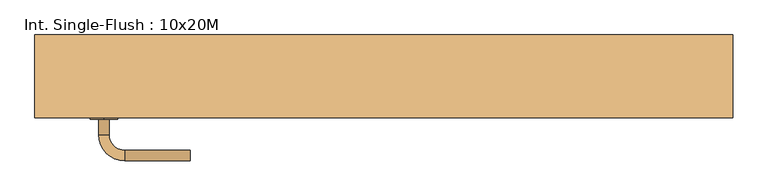
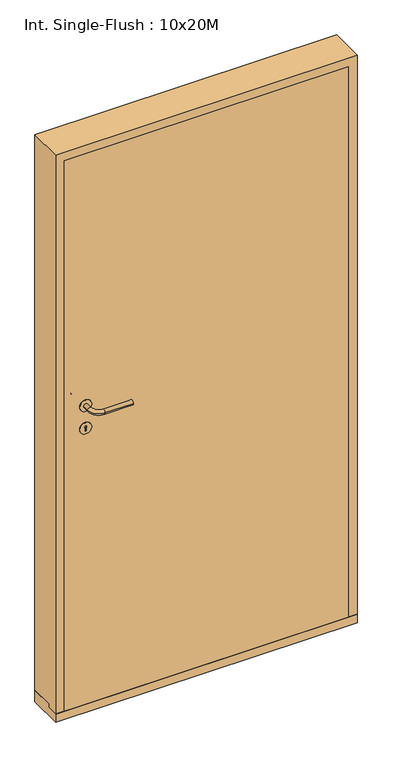
"""IFC4 building model written with IfcOpenShell, lengths in millimetres: door geometry, Int. Single-Flush : 10x20M."""

import ifcopenshell
import ifcopenshell.guid

model = None  # the IFC model being written
_history = None  # IfcOwnerHistory: only IFC2X3 demands one
_inside = {}  # id of a spatial element -> (the spatial element, [elements in it])
_under = {}  # id of a project, library or spatial element -> (it, [spatial elements below it])
_declared = {}  # id of a project -> (the project, [libraries it declares])
_typed = {}  # id of a type object -> (the type object, [elements of that type])
_made_of = {}  # id of a material, layer set ... -> (it, [elements and type objects made of it])


def new_model(schema):
    """Start an empty IFC model of exactly this schema.

    Asked for "IFC4X3", IfcOpenShell would pick the latest addendum, in which some entities
    have other attributes; the version numbers below select the first issue.
    IFC2X3 requires an IfcOwnerHistory on every rooted entity: one is made here for all.
    """
    global model, _history
    if schema == "IFC4X3":
        model = ifcopenshell.file(schema_version=(4, 3, 0, 0))
    else:
        model = ifcopenshell.file(schema=schema)
    _inside.clear()
    _under.clear()
    _declared.clear()
    _typed.clear()
    _made_of.clear()
    _history = None
    if model.schema == "IFC2X3":
        org = make("IfcOrganization", Name="unknown")
        user = make(
            "IfcPersonAndOrganization",
            ThePerson=make("IfcPerson", FamilyName="unknown"),
            TheOrganization=org,
        )
        app = make(
            "IfcApplication",
            ApplicationDeveloper=org,
            Version="unknown",
            ApplicationFullName="unknown",
            ApplicationIdentifier="unknown",
        )
        _history = make(
            "IfcOwnerHistory",
            OwningUser=user,
            OwningApplication=app,
            ChangeAction="ADDED",
            CreationDate=0,
        )
    return model


def make(cls, **values):
    """One entity of the class cls with the attributes given. An attribute that is None is left unset."""
    return model.create_entity(
        cls, **{name: value for name, value in values.items() if value is not None}
    )


def rooted(cls, **values):
    """An entity with a GlobalId (a new one), such as an element, a storey or a relation."""
    return make(cls, GlobalId=ifcopenshell.guid.new(), OwnerHistory=_history, **values)


def si_unit(unit_type, name, prefix=None):
    """IfcSIUnit, for example si_unit("LENGTHUNIT", "METRE", prefix="MILLI")."""
    return make("IfcSIUnit", UnitType=unit_type, Prefix=prefix, Name=name)


def assignment(units):
    """IfcUnitAssignment: the units of a project."""
    return None if units is None else make("IfcUnitAssignment", Units=units)


def point(xyz):
    """IfcCartesianPoint."""
    return None if xyz is None else make("IfcCartesianPoint", Coordinates=xyz)


def direction(xyz):
    """IfcDirection."""
    return None if xyz is None else make("IfcDirection", DirectionRatios=xyz)


def frame(location, z_axis=None, x_axis=None):
    """IfcAxis2Placement3D, a coordinate frame: its origin and axes. An axis left out is left unset."""
    return make(
        "IfcAxis2Placement3D",
        Location=point(location),
        Axis=direction(z_axis),
        RefDirection=direction(x_axis),
    )


def frame_2d(location, x_axis=None):
    """IfcAxis2Placement2D, a coordinate frame in the plane: its origin and x axis."""
    return make(
        "IfcAxis2Placement2D", Location=point(location), RefDirection=direction(x_axis)
    )


def origin():
    """The frame at (0, 0, 0) with its axes left unset."""
    return frame((0.0, 0.0, 0.0))


def place(relative_to, where):
    """IfcLocalPlacement: puts the frame where relative to a parent placement (None: the world)."""
    return make(
        "IfcLocalPlacement", PlacementRelTo=relative_to, RelativePlacement=where
    )


def context(
    kind, dimensions, precision=None, world=None, true_north=None, identifier=None
):
    """IfcGeometricRepresentationContext, for example the 3D "Model" context."""
    return make(
        "IfcGeometricRepresentationContext",
        ContextIdentifier=identifier,
        ContextType=kind,
        CoordinateSpaceDimension=dimensions,
        Precision=precision,
        WorldCoordinateSystem=world,
        TrueNorth=true_north,
    )


def project(units=None, contexts=None):
    """IfcProject with its units and contexts."""
    return rooted(
        "IfcProject",
        Name="project",
        RepresentationContexts=contexts,
        UnitsInContext=assignment(units),
    )


def spatial(cls, under=None, at=None, **own):
    """A site, building, storey or space (cls), placed at a placement, below another one or the project."""
    s = rooted(cls, ObjectPlacement=at, **own)
    if under is not None:
        _under.setdefault(under.id(), (under, []))[1].append(s)
    return s


def polyline(points):
    """IfcPolyline through the points."""
    return make("IfcPolyline", Points=[point(p) for p in points])


def circle_curve(where, radius):
    """IfcCircle in the frame where."""
    return make("IfcCircle", Position=where, Radius=radius)


def ellipse_curve(where, semi_axis1, semi_axis2):
    """IfcEllipse in the frame where."""
    return make(
        "IfcEllipse", Position=where, SemiAxis1=semi_axis1, SemiAxis2=semi_axis2
    )


def trimmed(basis, trim1, trim2, sense, master):
    """IfcTrimmedCurve: the piece of a basis curve between two trims."""
    return make(
        "IfcTrimmedCurve",
        BasisCurve=basis,
        Trim1=trim1,
        Trim2=trim2,
        SenseAgreement=sense,
        MasterRepresentation=master,
    )


def segment(curve, same_sense, transition):
    """IfcCompositeCurveSegment."""
    return make(
        "IfcCompositeCurveSegment",
        Transition=transition,
        SameSense=same_sense,
        ParentCurve=curve,
    )


def composite_curve(segments, self_intersect=None):
    """IfcCompositeCurve: segments joined end to end."""
    return make("IfcCompositeCurve", Segments=segments, SelfIntersect=self_intersect)


def outline(outer, holes=None, kind="AREA"):
    """IfcArbitraryClosedProfileDef: a profile drawn as a closed curve; with holes, ...WithVoids."""
    if holes is None:
        return make("IfcArbitraryClosedProfileDef", ProfileType=kind, OuterCurve=outer)
    return make(
        "IfcArbitraryProfileDefWithVoids",
        ProfileType=kind,
        OuterCurve=outer,
        InnerCurves=holes,
    )


def extrude(swept, where, along, depth):
    """IfcExtrudedAreaSolid: the profile swept, set in the frame where, extruded along a direction by depth."""
    return make(
        "IfcExtrudedAreaSolid",
        SweptArea=swept,
        Position=where,
        ExtrudedDirection=direction(along),
        Depth=depth,
    )


def faces_of(points, faces, orient=None, outer=None):
    """IfcFace entities. A face is a list of loops; a loop is a list of indices into points, from 0.

    orient and outer hold one flag for each loop. By default every Orientation is true, the
    first loop of a face is its IfcFaceOuterBound and the others are IfcFaceBound.
    """
    made = []
    for i, loops in enumerate(faces):
        bounds = []
        for j, loop in enumerate(loops):
            is_outer = j == 0 if outer is None else outer[i][j]
            bounds.append(
                make(
                    "IfcFaceOuterBound" if is_outer else "IfcFaceBound",
                    Bound=make("IfcPolyLoop", Polygon=[points[k] for k in loop]),
                    Orientation=True if orient is None else orient[i][j],
                )
            )
        made.append(make("IfcFace", Bounds=bounds))
    return made


def faceted_brep(points, faces, orient=None, outer=None, voids=None):
    """IfcFacetedBrep: a solid bounded by flat faces; with voids (closed shells), ...WithVoids."""
    shared = [point(p) for p in points]
    hull = make("IfcClosedShell", CfsFaces=faces_of(shared, faces, orient, outer))
    if voids is None:
        return make("IfcFacetedBrep", Outer=hull)
    return make(
        "IfcFacetedBrepWithVoids",
        Outer=hull,
        Voids=[
            make(cls, CfsFaces=faces_of(shared, fs, o, b)) for cls, fs, o, b in voids
        ],
    )


def shape(context_of_items, identifier, shape_type, items):
    """IfcShapeRepresentation: the items that make up one representation, for example the "Body"."""
    return make(
        "IfcShapeRepresentation",
        ContextOfItems=context_of_items,
        RepresentationIdentifier=identifier,
        RepresentationType=shape_type,
        Items=items,
    )


def source(mapping_origin, context_of_items, identifier, shape_type, items):
    """IfcRepresentationMap: a shape defined once, which mapped items show again and again."""
    return make(
        "IfcRepresentationMap",
        MappingOrigin=mapping_origin,
        MappedRepresentation=shape(context_of_items, identifier, shape_type, items),
    )


def transform(
    local_origin,
    x_axis=None,
    y_axis=None,
    z_axis=None,
    scale=None,
    scale2=None,
    scale3=None,
    uniform=True,
):
    """IfcCartesianTransformationOperator3D, or its non-uniform kind. x_axis, y_axis, z_axis: its Axis1, 2, 3."""
    if uniform:
        return make(
            "IfcCartesianTransformationOperator3D",
            Axis1=direction(x_axis),
            Axis2=direction(y_axis),
            LocalOrigin=point(local_origin),
            Scale=scale,
            Axis3=direction(z_axis),
        )
    return make(
        "IfcCartesianTransformationOperator3DnonUniform",
        Axis1=direction(x_axis),
        Axis2=direction(y_axis),
        LocalOrigin=point(local_origin),
        Scale=scale,
        Axis3=direction(z_axis),
        Scale2=scale2,
        Scale3=scale3,
    )


def mapped(mapping_source, mapping_target):
    """IfcMappedItem: shows the shape of a source again, moved by a transform."""
    return make(
        "IfcMappedItem", MappingSource=mapping_source, MappingTarget=mapping_target
    )


def made_of(thing, what):
    """Note that an element or type object is made of a material, layer set ...; save() writes the relation."""
    if what is not None:
        _made_of.setdefault(what.id(), (what, []))[1].append(thing)
    return thing


def element(
    cls,
    number,
    at=None,
    inside=None,
    cuts=None,
    type_object=None,
    material=None,
    context=None,
    identifier="Body",
    shape_type=None,
    held_by="IfcProductDefinitionShape",
    body=None,
    shapes=None,
    **own,
):
    """One element of the class cls, such as IfcWall. Its Tag is "e" and its number.

    at: its placement. inside: the storey or other place that contains it. cuts: it is an
    opening in that element (IfcRelVoidsElement). A single representation is given by context,
    identifier, shape_type and body (its items); several are given by shapes. held_by: the class
    of the entity that holds the representations. save() writes the other relations.
    """
    e = rooted(cls, Tag="e%d" % number, ObjectPlacement=at, **own)
    if body is not None:
        shapes = [shape(context, identifier, shape_type, body)]
    if shapes is not None:
        e.Representation = make(held_by, Representations=shapes)
    if inside is not None:
        _inside.setdefault(inside.id(), (inside, []))[1].append(e)
    if cuts is not None:
        rooted(
            "IfcRelVoidsElement", RelatingBuildingElement=cuts, RelatedOpeningElement=e
        )
    if type_object is not None:
        _typed.setdefault(type_object.id(), (type_object, []))[1].append(e)
    return made_of(e, material)


def aggregate(whole, parts):
    """IfcRelAggregates: a whole, such as a stair, and the parts it consists of."""
    return rooted("IfcRelAggregates", RelatingObject=whole, RelatedObjects=parts)


def save(model, path):
    """Write the relations noted so far, then the file.

    IfcRelAggregates (storeys below a building ...), IfcRelContainedInSpatialStructure (elements
    in a storey), IfcRelDefinesByType, IfcRelAssociatesMaterial and IfcRelDeclares: one each for
    every whole, place, type object, material and project.
    """
    for whole, parts in _under.values():
        aggregate(whole, parts)
    for where, things in _inside.values():
        rooted(
            "IfcRelContainedInSpatialStructure",
            RelatedElements=things,
            RelatingStructure=where,
        )
    for kind, things in _typed.values():
        rooted("IfcRelDefinesByType", RelatedObjects=things, RelatingType=kind)
    for what, things in _made_of.values():
        rooted("IfcRelAssociatesMaterial", RelatedObjects=things, RelatingMaterial=what)
    for by, libraries in _declared.values():
        rooted("IfcRelDeclares", RelatingContext=by, RelatedDefinitions=libraries)
    model.write(path)


def plane_surface(at):
    """IfcPlane: the flat surface through the origin of the frame at, square to its z axis."""
    return make("IfcPlane", Position=at)


def cylinder_surface(at, radius):
    """IfcCylindricalSurface: all points at the distance radius from the z axis of the frame at."""
    return make("IfcCylindricalSurface", Position=at, Radius=radius)


def revolved_surface(curve, axis_point, axis_direction):
    """IfcSurfaceOfRevolution: the curve turned about the line through axis_point along axis_direction."""
    return make(
        "IfcSurfaceOfRevolution",
        SweptCurve=make("IfcArbitraryOpenProfileDef", ProfileType="CURVE", Curve=curve),
        AxisPosition=make("IfcAxis1Placement", Location=point(axis_point), Axis=direction(axis_direction)),
    )


def advanced_brep(points, edges, surfaces, faces):
    """IfcAdvancedBrep: a solid bounded by faces that lie on surfaces and meet in shared edges.

    An edge is (start, end): straight between two places in points (the first is 0);
    or (start, end, curve); or (start, end, curve, False) where it runs against its curve.
    A face is (place in surfaces, loops), or (place, loops, False) where it looks against
    its surface's normal. A loop lists edges by number (the first is 1), with a minus sign
    where the edge is run from its end to its start. The first loop is the outer one.
    """
    corners = [point(p) for p in points]
    vertices = [make("IfcVertexPoint", VertexGeometry=c) for c in corners]
    made = []
    for start, end, *more in edges:
        made.append(
            make(
                "IfcEdgeCurve",
                EdgeStart=vertices[start],
                EdgeEnd=vertices[end],
                EdgeGeometry=more[0] if more else make("IfcPolyline", Points=[corners[start], corners[end]]),
                SameSense=more[1] if len(more) > 1 else True,
            )
        )
    hull = []
    for where, loops, *sense in faces:
        bounds = []
        for j, loop in enumerate(loops):
            ring = [make("IfcOrientedEdge", EdgeElement=made[abs(k) - 1], Orientation=k > 0) for k in loop]
            bounds.append(
                make(
                    "IfcFaceOuterBound" if j == 0 else "IfcFaceBound",
                    Bound=make("IfcEdgeLoop", EdgeList=ring),
                    Orientation=True,
                )
            )
        hull.append(make("IfcAdvancedFace", Bounds=bounds, FaceSurface=surfaces[where], SameSense=sense[0] if sense else True))
    return make("IfcAdvancedBrep", Outer=make("IfcClosedShell", CfsFaces=hull))


def int_single_flush_10x20m_68751a9d(model_context):
    return source(origin(), model_context, "Body", "SolidModel", [
        extrude(outline(composite_curve([segment(trimmed(circle_curve(frame_2d((1090.0, -406.0)), 20.0), [point((1070.0, -406.0))], [point((1110.0, -406.0))], False, "CARTESIAN"), True, "CONTINUOUS"), segment(trimmed(circle_curve(frame_2d((1090.0, -406.0)), 20.0), [point((1110.0, -406.0))], [point((1070.0, -406.0))], False, "CARTESIAN"), True, "CONTINUOUS")], self_intersect=False)), frame((0.0, -62.0, 0.0), z_axis=(0.0, 1.0, 0.0), x_axis=(0.0, 0.0, 1.0)), (0.0, 0.0, 1.0), 2.0),
        advanced_brep(
        [(-413.5, -62.0, 1090.0), (-398.5, -62.0, 1090.0), (-398.5, -84.5, 1090.0), (-413.5, -84.5, 1090.0), (-376.0, -107.0, 1090.0), (-376.0, -122.0, 1090.0), (-281.0, -107.0, 1090.0), (-281.0, -122.0, 1090.0)],
        [
            (0, 1, circle_curve(frame((-406.0, -62.0, 1090.0), z_axis=(0.0, 1.0, 0.0), x_axis=(1.0, 0.0, 0.0)), 7.5)),
            (1, 0, circle_curve(frame((-406.0, -62.0, 1090.0), z_axis=(0.0, 1.0, 0.0), x_axis=(1.0, 0.0, 0.0)), 7.5)),
            (1, 2),
            (2, 3, circle_curve(frame((-406.0, -84.5, 1090.0), z_axis=(0.0, 1.0, 0.0), x_axis=(1.0, 0.0, 0.0)), 7.5)),
            (3, 0),
            (3, 2, circle_curve(frame((-406.0, -84.5, 1090.0), z_axis=(0.0, 1.0, 0.0), x_axis=(1.0, 0.0, 0.0)), 7.5)),
            (4, 5, circle_curve(frame((-376.0, -114.5, 1090.0), z_axis=(-1.0, 0.0, 0.0), x_axis=(0.0, 1.0, 0.0)), 7.5)),
            (5, 3, circle_curve(frame((-376.0, -84.5, 1090.0), z_axis=(0.0, 0.0, -1.0), x_axis=(-1.0, 0.0, 0.0)), 37.5)),
            (2, 4, circle_curve(frame((-376.0, -84.5, 1090.0), z_axis=(0.0, 0.0, 1.0), x_axis=(-1.0, 0.0, 0.0)), 22.5)),
            (5, 4, circle_curve(frame((-376.0, -114.5, 1090.0), z_axis=(-1.0, 0.0, 0.0), x_axis=(0.0, 1.0, 0.0)), 7.5)),
            (4, 6),
            (6, 7, circle_curve(frame((-281.0, -114.5, 1090.0), z_axis=(-1.0, 0.0, 0.0), x_axis=(0.0, 1.0, 0.0)), 7.5)),
            (7, 5),
            (7, 6, circle_curve(frame((-281.0, -114.5, 1090.0), z_axis=(-1.0, 0.0, 0.0), x_axis=(0.0, 1.0, 0.0)), 7.5)),
        ],
        [
            plane_surface(frame((-406.0, -62.0, 1090.0), z_axis=(0.0, 1.0, 0.0), x_axis=(0.0, 0.0, -1.0))),
            cylinder_surface(frame((-406.0, -62.0, 1090.0), z_axis=(0.0, 1.0, 0.0), x_axis=(1.0, 0.0, 0.0)), 7.5),
            revolved_surface(trimmed(ellipse_curve(frame((-406.0, -84.5, 1090.0), z_axis=(0.0, -1.0, 0.0), x_axis=(1.0, 0.0, 0.0)), 7.5, 7.5), [point((-413.5, -84.5, 1090.0))], [point((-398.5, -84.5, 1090.0))], True, "CARTESIAN"), (-376.0, -84.5, 1090.0), (0.0, 0.0, -1.0)),
            revolved_surface(trimmed(ellipse_curve(frame((-406.0, -84.5, 1090.0), z_axis=(0.0, -1.0, 0.0), x_axis=(1.0, 0.0, 0.0)), 7.5, 7.5), [point((-398.5, -84.5, 1090.0))], [point((-413.5, -84.5, 1090.0))], True, "CARTESIAN"), (-376.0, -84.5, 1090.0), (0.0, 0.0, -1.0)),
            cylinder_surface(frame((-376.0, -114.5, 1090.0), z_axis=(-1.0, 0.0, 0.0), x_axis=(0.0, 1.0, 0.0)), 7.5),
            plane_surface(frame((-281.0, -114.5, 1090.0), z_axis=(1.0, 0.0, 0.0), x_axis=(0.0, 0.0, -1.0))),
        ],
        [
            (0, [[1, 2]]),
            (1, [[3, 4, 5, -2]]),
            (1, [[-5, 6, -3, -1]]),
            (2, [[7, 8, -4, 9]]),
            (3, [[10, -9, -6, -8]]),
            (4, [[11, 12, 13, -7]]),
            (4, [[-13, 14, -11, -10]]),
            (5, [[-12, -14]]),
        ],
    ),
        extrude(outline(composite_curve([segment(trimmed(circle_curve(frame_2d((1010.0, -406.0)), 20.0), [point((990.0, -406.0))], [point((1030.0, -406.0))], False, "CARTESIAN"), True, "CONTINUOUS"), segment(trimmed(circle_curve(frame_2d((1010.0, -406.0)), 20.0), [point((1030.0, -406.0))], [point((990.0, -406.0))], False, "CARTESIAN"), True, "CONTINUOUS")], self_intersect=False), holes=[composite_curve([segment(trimmed(circle_curve(frame_2d((1015.0, -406.0)), 3.0), [point((1012.4019238, -407.5))], [point((1012.4019238, -404.5))], True, "CARTESIAN"), True, "CONTINUOUS"), segment(polyline([(1012.4019238, -404.5), (1000.0, -404.5), (1000.0, -407.5), (1012.4019238, -407.5)]), True, "CONTINUOUS")], self_intersect=False)]), frame((0.0, -62.0, 0.0), z_axis=(0.0, 1.0, 0.0), x_axis=(0.0, 0.0, 1.0)), (0.0, 0.0, 1.0), 2.0),
        extrude(outline(composite_curve([segment(trimmed(circle_curve(frame_2d((1090.0, -406.0)), 20.0), [point((1070.0, -406.0))], [point((1110.0, -406.0))], False, "CARTESIAN"), True, "CONTINUOUS"), segment(trimmed(circle_curve(frame_2d((1090.0, -406.0)), 20.0), [point((1110.0, -406.0))], [point((1070.0, -406.0))], False, "CARTESIAN"), True, "CONTINUOUS")], self_intersect=False)), frame((0.0, -20.0, 0.0), z_axis=(0.0, 1.0, 0.0), x_axis=(0.0, 0.0, 1.0)), (0.0, 0.0, 1.0), 2.0),
        advanced_brep(
        [(-413.5, -18.0, 1090.0), (-398.5, -18.0, 1090.0), (-413.5, 4.5, 1090.0), (-398.5, 4.5, 1090.0), (-376.0, 27.0, 1090.0), (-376.0, 42.0, 1090.0), (-281.0, 42.0, 1090.0), (-281.0, 27.0, 1090.0)],
        [
            (0, 1, circle_curve(frame((-406.0, -18.0, 1090.0), z_axis=(0.0, -1.0, 0.0), x_axis=(1.0, 0.0, 0.0)), 7.5)),
            (1, 0, circle_curve(frame((-406.0, -18.0, 1090.0), z_axis=(0.0, -1.0, 0.0), x_axis=(1.0, 0.0, 0.0)), 7.5)),
            (0, 2),
            (2, 3, circle_curve(frame((-406.0, 4.5, 1090.0), z_axis=(0.0, -1.0, 0.0), x_axis=(1.0, 0.0, 0.0)), 7.5)),
            (3, 1),
            (3, 2, circle_curve(frame((-406.0, 4.5, 1090.0), z_axis=(0.0, -1.0, 0.0), x_axis=(1.0, 0.0, 0.0)), 7.5)),
            (4, 3, circle_curve(frame((-376.0, 4.5, 1090.0), z_axis=(0.0, 0.0, 1.0), x_axis=(-1.0, 0.0, 0.0)), 22.5)),
            (2, 5, circle_curve(frame((-376.0, 4.5, 1090.0), z_axis=(0.0, 0.0, -1.0), x_axis=(-1.0, 0.0, 0.0)), 37.5)),
            (5, 4, circle_curve(frame((-376.0, 34.5, 1090.0), z_axis=(-1.0, 0.0, 0.0), x_axis=(0.0, -1.0, 0.0)), 7.5)),
            (4, 5, circle_curve(frame((-376.0, 34.5, 1090.0), z_axis=(-1.0, 0.0, 0.0), x_axis=(0.0, -1.0, 0.0)), 7.5)),
            (5, 6),
            (6, 7, circle_curve(frame((-281.0, 34.5, 1090.0), z_axis=(-1.0, 0.0, 0.0), x_axis=(0.0, -1.0, 0.0)), 7.5)),
            (7, 4),
            (7, 6, circle_curve(frame((-281.0, 34.5, 1090.0), z_axis=(-1.0, 0.0, 0.0), x_axis=(0.0, -1.0, 0.0)), 7.5)),
        ],
        [
            plane_surface(frame((-406.0, -18.0, 1090.0), z_axis=(0.0, -1.0, 0.0), x_axis=(0.0, 0.0, -1.0))),
            cylinder_surface(frame((-406.0, -18.0, 1090.0), z_axis=(0.0, -1.0, 0.0), x_axis=(1.0, 0.0, 0.0)), 7.5),
            revolved_surface(trimmed(ellipse_curve(frame((-406.0, 4.5, 1090.0), z_axis=(0.0, -1.0, 0.0), x_axis=(1.0, 0.0, 0.0)), 7.5, 7.5), [point((-413.5, 4.5, 1090.0))], [point((-398.5, 4.5, 1090.0))], True, "CARTESIAN"), (-376.0, 4.5, 1090.0), (0.0, 0.0, -1.0)),
            revolved_surface(trimmed(ellipse_curve(frame((-406.0, 4.5, 1090.0), z_axis=(0.0, -1.0, 0.0), x_axis=(1.0, 0.0, 0.0)), 7.5, 7.5), [point((-398.5, 4.5, 1090.0))], [point((-413.5, 4.5, 1090.0))], True, "CARTESIAN"), (-376.0, 4.5, 1090.0), (0.0, 0.0, -1.0)),
            cylinder_surface(frame((-376.0, 34.5, 1090.0), z_axis=(-1.0, 0.0, 0.0), x_axis=(0.0, -1.0, 0.0)), 7.5),
            plane_surface(frame((-281.0, 34.5, 1090.0), z_axis=(1.0, 0.0, 0.0), x_axis=(0.0, 0.0, -1.0))),
        ],
        [
            (0, [[1, 2]]),
            (1, [[-1, 3, 4, 5]]),
            (1, [[-2, -5, 6, -3]]),
            (2, [[7, -4, 8, 9]]),
            (3, [[-8, -6, -7, 10]]),
            (4, [[-9, 11, 12, 13]]),
            (4, [[-10, -13, 14, -11]]),
            (5, [[-14, -12]]),
        ],
    ),
        extrude(outline(composite_curve([segment(trimmed(circle_curve(frame_2d((1010.0, -406.0)), 20.0), [point((990.0, -406.0))], [point((1030.0, -406.0))], False, "CARTESIAN"), True, "CONTINUOUS"), segment(trimmed(circle_curve(frame_2d((1010.0, -406.0)), 20.0), [point((1030.0, -406.0))], [point((990.0, -406.0))], False, "CARTESIAN"), True, "CONTINUOUS")], self_intersect=False), holes=[composite_curve([segment(trimmed(circle_curve(frame_2d((1015.0, -406.0)), 3.0), [point((1012.4019238, -407.5))], [point((1012.4019238, -404.5))], True, "CARTESIAN"), True, "CONTINUOUS"), segment(polyline([(1012.4019238, -404.5), (1000.0, -404.5), (1000.0, -407.5), (1012.4019238, -407.5)]), True, "CONTINUOUS")], self_intersect=False)]), frame((0.0, -20.0, 0.0), z_axis=(0.0, 1.0, 0.0), x_axis=(0.0, 0.0, 1.0)), (0.0, 0.0, 1.0), 2.0),
        extrude(outline(polyline([(476.0, -20.0), (476.0, -60.0), (-476.0, -60.0), (-476.0, -20.0), (476.0, -20.0)])), frame((0.0, 0.0, 30.0), z_axis=(0.0, 0.0, 1.0), x_axis=(1.0, 0.0, 0.0)), (0.0, 0.0, 1.0), 1952.0),
        extrude(outline(polyline([(-20.0, 42.0), (60.0, 42.0), (60.0, 0.0), (-60.0, 0.0), (-60.0, 30.0), (-20.0, 30.0), (-20.0, 42.0)])), frame((-506.0, 0.0, 0.0), z_axis=(1.0, 0.0, 0.0), x_axis=(0.0, 1.0, 0.0)), (0.0, 0.0, 1.0), 1012.0),
        faceted_brep([(-476.0, -20.0, 1982.0), (-476.0, -20.0, 42.0), (-464.0, -20.0, 42.0), (-464.0, -20.0, 1970.0), (464.0, -20.0, 1970.0), (464.0, -20.0, 42.0), (476.0, -20.0, 42.0), (476.0, -20.0, 1982.0), (-476.0, -60.0, 1982.0), (-476.0, -60.0, 30.0), (-476.0, -20.0, 30.0), (-506.0, -20.0, 30.0), (-506.0, -20.0, 42.0), (506.0, -20.0, 42.0), (506.0, -20.0, 30.0), (476.0, -20.0, 30.0), (-506.0, -60.0, 30.0), (506.0, -60.0, 30.0), (476.0, -60.0, 30.0), (-506.0, -60.0, 2012.0), (476.0, -60.0, 1982.0), (506.0, -60.0, 2012.0), (464.0, 60.0, 42.0), (506.0, 60.0, 42.0), (-506.0, 60.0, 42.0), (-464.0, 60.0, 42.0), (464.0, 60.0, 1970.0), (-464.0, 60.0, 1970.0), (-506.0, 60.0, 2012.0), (506.0, 60.0, 2012.0)], [[[0, 1, 2, 3, 4, 5, 6, 7]], [[8, 9, 10, 1, 0]], [[1, 10, 11, 12]], [[13, 14, 15, 6]], [[10, 9, 16, 11]], [[14, 17, 18, 15]], [[19, 16, 9, 8, 20, 18, 17, 21]], [[7, 6, 15, 18, 20]], [[6, 5, 22, 23, 13]], [[12, 24, 25, 2, 1]], [[26, 22, 5, 4]], [[3, 2, 25, 27]], [[27, 25, 24, 28, 29, 23, 22, 26]], [[21, 17, 14, 13, 23, 29]], [[28, 24, 12, 11, 16, 19]], [[0, 7, 20, 8]], [[3, 27, 26, 4]], [[28, 19, 21, 29]]]),
    ])


if __name__ == "__main__":
    model = new_model("IFC4")
    model_context = context("Model", 3, world=origin())
    ifc_project = project(units=[si_unit("LENGTHUNIT", "METRE", prefix="MILLI")], contexts=[model_context])
    site = spatial("IfcSite", under=ifc_project)
    building = spatial("IfcBuilding", under=site)
    placement = place(None, origin())
    int_single_flush_10x20m_shape = int_single_flush_10x20m_68751a9d(model_context)
    element("IfcDoor", 1, ObjectType="Int. Single-Flush : 10x20M", at=placement, inside=building, context=model_context, shape_type="MappedRepresentation", body=[
        mapped(int_single_flush_10x20m_shape, transform((0.0, 0.0, 0.0), x_axis=(1.0, 0.0, 0.0), y_axis=(0.0, 1.0, 0.0), z_axis=(0.0, 0.0, 1.0))),
    ])
    save(model, "model.ifc")

# Revit data of these elements
# Type "Int. Single-Flush : 10x20M"
#   Type Mark = "73"
#   Sound Rating = ""
#   Hinge Side [instance default] = ""
#   Creator Organization [instance default] = "© Danish Educational Content"
#   Creator Name [instance default] = "© Erik Falck Jørgensen"
#   Creator Build [instance default] = "2017.0801.0"
#   Analytic Construction = "<None>"
#   length#5 = 1012 mm
#   length#3 = 42 mm
#   length#2b = 12 mm
#   length#2a = 0 mm
#   length#2 = 0 mm
#   length#1a = 12 mm
#   length#1 = 0 mm
#   length#4 = 30 mm
#   Thickness = 40 mm
#   Seal Width = 12 mm
#   Rough Width = 1012 mm
#   Rough Height = 2012 mm
#   Rabbet Depth = 40 mm
#   Interior Distance [instance default] = 0 mm
#   Height = 1988 mm
#   Width = 988 mm
#   Handle From Side = 100 mm
#   Handle From Bottom = 1090 mm
#   Exterior Direction [instance default] = 0.00°
#   Case Depth [instance default] = 200 mm
#   Case Width = 30 mm
#   Rabbet Width = 12 mm
#   Exterior Distance [instance default] = 0 mm
#   Bottom Seal = 12 mm
#   Threshold = yes
#   Sealing = no
#   Hinging = yes
#   Wall Closure = 1
#   Door Panel = no
#   Panel = none
#   Handle Finish = none
#   Handle = element 510752
#   Case/Transom = none
#   Function = (empty or 0)
#   Assembly Code = ""
# Element 1 (IfcDoor, "Int. Single-Flush : 10x20M")
#   Case Depth = 120 mm
#   Materials on its faces: "Stainless Steel, Polished", "Default Frame/Mullion (Interior/Exterior)", "Default Door Panel (Exterior/Interior)"
# Materials
#   "Stainless Steel, Polished": class "Metal", colour RGB 180 180 180, transparency 0, Description = "Rustfri stål, poleret", Cost = 0
#   "Default Frame/Mullion (Interior/Exterior)": class "Generic", colour RGB 205 205 205, transparency 0, Description = "Udefineret karm/ramme materiale", Cost = 0
#   "Default Door Panel (Exterior/Interior)": class "Generic", colour RGB 205 205 205, transparency 0, Description = "Udefineret dørplade materiale", Cost = 0
